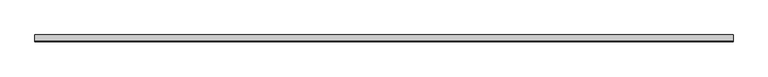
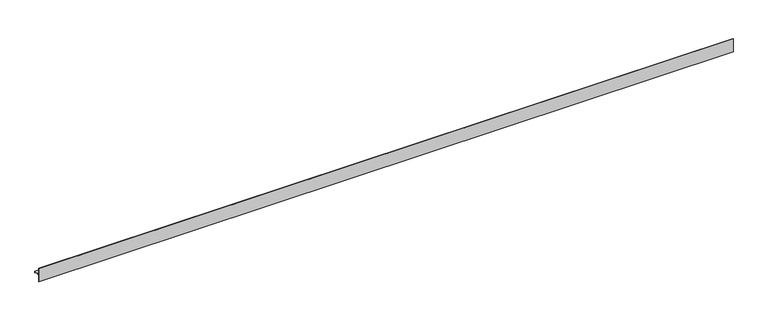
"""IFC4 building model written with IfcOpenShell, lengths in millimetres: proxy geometry, Metal profile002 527 : Metal profile002 527."""

from ifc_helpers import new_model, si_unit, frame, origin, place, context, project, spatial, polyline, outline, extrude, source, transform, mapped, element, save


def generic_models_88e4c6c3(model_context):
    return source(origin(), model_context, "Body", "SweptSolid", [
        extrude(outline(polyline([(10460.9050834, 40757.6682813), (10443.9411354, 40757.6682813), (10443.9411354, 40738.6182812), (10442.6711354, 40738.6182812), (10442.6711354, 40777.9882813), (10443.9411354, 40777.9882813), (10443.9411354, 40758.9382813), (10462.1750834, 40758.9382813), (10462.1750834, 40754.1884812), (10460.9050834, 40754.1884812), (10460.9050834, 40757.6682813)])), frame((3694.2883192, 0.0, 0.0), z_axis=(1.0, 0.0, 0.0), x_axis=(0.0, 1.0, 0.0)), (0.0, 0.0, 1.0), 2000.0),
    ])


if __name__ == "__main__":
    model = new_model("IFC4")
    model_context = context("Model", 3, world=origin())
    ifc_project = project(units=[si_unit("LENGTHUNIT", "METRE", prefix="MILLI")], contexts=[model_context])
    site = spatial("IfcSite", under=ifc_project)
    building = spatial("IfcBuilding", under=site)
    placement = place(None, origin())
    generic_models_shape = generic_models_88e4c6c3(model_context)
    element("IfcBuildingElementProxy", 1, Name="Metal profile002 527 : Metal profile002 527", ObjectType="Metal profile002 527 : Metal profile002 527", at=placement, inside=building, context=model_context, shape_type="MappedRepresentation", body=[
        mapped(generic_models_shape, transform((0.0, 0.0, 0.0), x_axis=(1.0, 0.0, 0.0), y_axis=(0.0, 1.0, 0.0), z_axis=(0.0, 0.0, 1.0))),
    ])
    save(model, "model.ifc")

# Revit data of these elements
# Type "Metal profile002 527 : Metal profile002 527"
#   NameOverride = "Metal profile002"
# Element 1 (IfcBuildingElementProxy, "Metal profile002 527 : Metal profile002 527")
#   Materials on its faces: "16 GA. COPPER VENTED T REVEAL BEAD"
# Materials
#   "16 GA. COPPER VENTED T REVEAL BEAD": class "Unassigned", colour RGB 255 227 10, transparency 0
